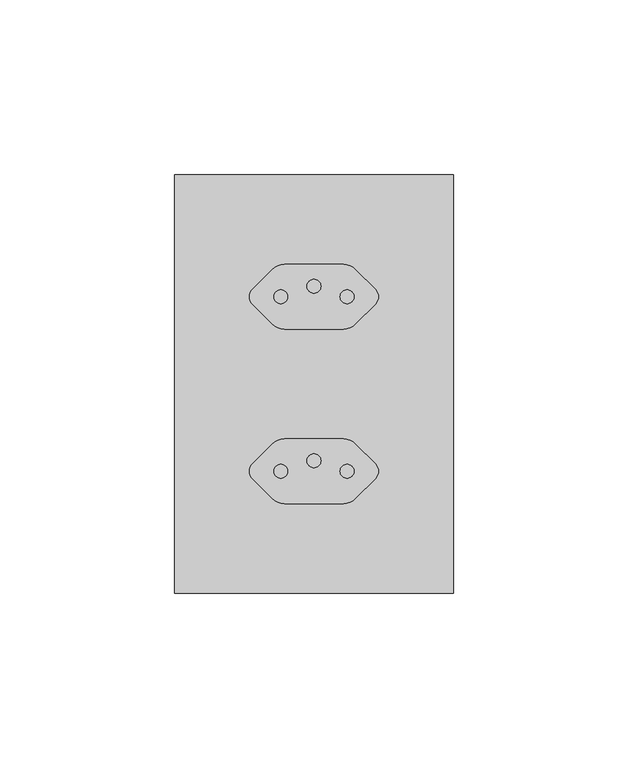
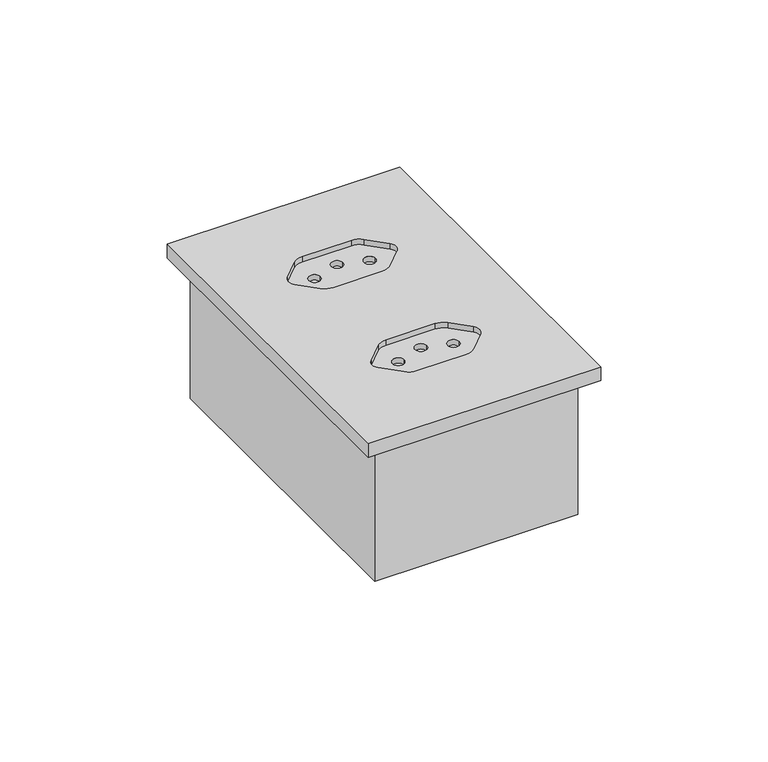
"""IFC4 building model written with IfcOpenShell, lengths in millimetres: proxy geometry, CAIXA VERTICE V7 : Tomada 10A 2s."""

from ifc_helpers import new_model, si_unit, frame, origin, place, context, project, spatial, polyline, circle_curve, faceted_brep, source, transform, mapped, element, save
from ifc_brep_helpers import plane_surface, revolved_surface, advanced_brep


def electrical_fixtures_84a19cd9(model_context):
    return source(origin(), model_context, "Body", "SolidModel", [
        faceted_brep([(33.0, 947.0, -48.0), (33.0, 1053.0, -48.0), (-33.0, 1053.0, -48.0), (-33.0, 947.0, -48.0), (35.0, 1055.0, -50.0), (35.0, 945.0, -50.0), (-35.0, 945.0, -50.0), (-35.0, 1055.0, -50.0), (-35.0, 1055.0, 0.0), (35.0, 1055.0, 0.0), (-35.0, 945.0, 0.0), (35.0, 945.0, 0.0), (33.0, 1053.0, 0.0), (33.0, 947.0, 0.0), (-33.0, 947.0, 0.0), (-33.0, 1053.0, 0.0)], [[[0, 1, 2, 3]], [[4, 5, 6, 7]], [[4, 7, 8, 9]], [[8, 7, 6, 10]], [[10, 6, 5, 11]], [[11, 5, 4, 9]], [[9, 8, 10, 11], [12, 13, 14, 15]], [[13, 12, 1, 0]], [[14, 13, 0, 3]], [[15, 14, 3, 2]], [[12, 15, 2, 1]]]),
        advanced_brep(
        [(40.0, 1060.0, 5.0), (-40.0, 1060.0, 5.0), (-40.0, 940.0, 5.0), (40.0, 940.0, 5.0), (8.4215729, 1015.75, 5.0), (-8.4215729, 1015.75, 5.0), (-11.9571068, 1017.2144661, 5.0), (-17.6213203, 1022.8786797, 5.0), (-17.6213203, 1027.1213203, 5.0), (-11.9571068, 1032.7855339, 5.0), (-8.4215729, 1034.25, 5.0), (8.4215729, 1034.25, 5.0), (11.9571068, 1032.7855339, 5.0), (17.6213203, 1027.1213203, 5.0), (17.6213203, 1022.8786797, 5.0), (11.9571068, 1017.2144661, 5.0), (8.4215729, 965.75, 5.0), (-8.4215729, 965.75, 5.0), (-11.9571068, 967.2144661, 5.0), (-17.6213203, 972.8786797, 5.0), (-17.6213203, 977.1213203, 5.0), (-11.9571068, 982.7855339, 5.0), (-8.4215729, 984.25, 5.0), (8.4215729, 984.25, 5.0), (11.9571068, 982.7855339, 5.0), (17.6213203, 977.1213203, 5.0), (17.6213203, 972.8786797, 5.0), (11.9571068, 967.2144661, 5.0), (-40.0, 1060.0, 0.0), (40.0, 1060.0, 0.0), (40.0, 940.0, 0.0), (-40.0, 940.0, 0.0), (8.4215729, 1015.75, 3.0), (11.9571068, 1017.2144661, 3.0), (17.6213203, 1022.8786797, 3.0), (17.6213203, 1027.1213203, 3.0), (11.9571068, 1032.7855339, 3.0), (8.4215729, 1034.25, 3.0), (-8.4215729, 1034.25, 3.0), (-11.9571068, 1032.7855339, 3.0), (-17.6213203, 1027.1213203, 3.0), (-17.6213203, 1022.8786797, 3.0), (-11.9571068, 1017.2144661, 3.0), (-8.4215729, 1015.75, 3.0), (-7.5, 1025.0, 3.0), (-11.5, 1025.0, 3.0), (11.5, 1025.0, 3.0), (7.5, 1025.0, 3.0), (2.0, 1028.0, 3.0), (-2.0, 1028.0, 3.0), (-11.5, 1025.0, 1.0), (-7.5, 1025.0, 1.0), (7.5, 1025.0, 1.0), (11.5, 1025.0, 1.0), (-2.0, 1028.0, 1.0), (2.0, 1028.0, 1.0), (8.4215729, 965.75, 3.0), (11.9571068, 967.2144661, 3.0), (17.6213203, 972.8786797, 3.0), (17.6213203, 977.1213203, 3.0), (11.9571068, 982.7855339, 3.0), (8.4215729, 984.25, 3.0), (-8.4215729, 984.25, 3.0), (-11.9571068, 982.7855339, 3.0), (-17.6213203, 977.1213203, 3.0), (-17.6213203, 972.8786797, 3.0), (-11.9571068, 967.2144661, 3.0), (-8.4215729, 965.75, 3.0), (-7.5, 975.0, 3.0), (-11.5, 975.0, 3.0), (11.5, 975.0, 3.0), (7.5, 975.0, 3.0), (2.0, 978.0, 3.0), (-2.0, 978.0, 3.0), (-11.5, 975.0, 1.0), (-7.5, 975.0, 1.0), (7.5, 975.0, 1.0), (11.5, 975.0, 1.0), (-2.0, 978.0, 1.0), (2.0, 978.0, 1.0)],
        [
            (0, 1),
            (1, 2),
            (2, 3),
            (3, 0),
            (4, 5),
            (5, 6, circle_curve(frame((-8.4215729, 1020.75, 5.0), z_axis=(0.0, 0.0, -1.0), x_axis=(-1.0, 0.0, 0.0)), 5.0)),
            (6, 7),
            (7, 8, circle_curve(frame((-15.5, 1025.0, 5.0), z_axis=(0.0, 0.0, -1.0), x_axis=(-1.0, 0.0, 0.0)), 3.0)),
            (8, 9),
            (9, 10, circle_curve(frame((-8.4215729, 1029.25, 5.0), z_axis=(0.0, 0.0, -1.0), x_axis=(-1.0, 0.0, 0.0)), 5.0)),
            (10, 11),
            (11, 12, circle_curve(frame((8.4215729, 1029.25, 5.0), z_axis=(0.0, 0.0, -1.0), x_axis=(-1.0, 0.0, 0.0)), 5.0)),
            (12, 13),
            (13, 14, circle_curve(frame((15.5, 1025.0, 5.0), z_axis=(0.0, 0.0, -1.0), x_axis=(-1.0, 0.0, 0.0)), 3.0)),
            (14, 15),
            (15, 4, circle_curve(frame((8.4215729, 1020.75, 5.0), z_axis=(0.0, 0.0, -1.0), x_axis=(-1.0, 0.0, 0.0)), 5.0)),
            (16, 17),
            (17, 18, circle_curve(frame((-8.4215729, 970.75, 5.0), z_axis=(0.0, 0.0, -1.0), x_axis=(-1.0, 0.0, 0.0)), 5.0)),
            (18, 19),
            (19, 20, circle_curve(frame((-15.5, 975.0, 5.0), z_axis=(0.0, 0.0, -1.0), x_axis=(-1.0, 0.0, 0.0)), 3.0)),
            (20, 21),
            (21, 22, circle_curve(frame((-8.4215729, 979.25, 5.0), z_axis=(0.0, 0.0, -1.0), x_axis=(-1.0, 0.0, 0.0)), 5.0)),
            (22, 23),
            (23, 24, circle_curve(frame((8.4215729, 979.25, 5.0), z_axis=(0.0, 0.0, -1.0), x_axis=(-1.0, 0.0, 0.0)), 5.0)),
            (24, 25),
            (25, 26, circle_curve(frame((15.5, 975.0, 5.0), z_axis=(0.0, 0.0, -1.0), x_axis=(-1.0, 0.0, 0.0)), 3.0)),
            (26, 27),
            (27, 16, circle_curve(frame((8.4215729, 970.75, 5.0), z_axis=(0.0, 0.0, -1.0), x_axis=(-1.0, 0.0, 0.0)), 5.0)),
            (28, 29),
            (29, 30),
            (30, 31),
            (31, 28),
            (0, 29),
            (28, 1),
            (31, 2),
            (30, 3),
            (32, 33, circle_curve(frame((8.4215729, 1020.75, 3.0), z_axis=(0.0, 0.0, 1.0), x_axis=(-1.0, 0.0, 0.0)), 5.0)),
            (33, 34),
            (34, 35, circle_curve(frame((15.5, 1025.0, 3.0), z_axis=(0.0, 0.0, 1.0), x_axis=(-1.0, 0.0, 0.0)), 3.0)),
            (35, 36),
            (36, 37, circle_curve(frame((8.4215729, 1029.25, 3.0), z_axis=(0.0, 0.0, 1.0), x_axis=(-1.0, 0.0, 0.0)), 5.0)),
            (37, 38),
            (38, 39, circle_curve(frame((-8.4215729, 1029.25, 3.0), z_axis=(0.0, 0.0, 1.0), x_axis=(-1.0, 0.0, 0.0)), 5.0)),
            (39, 40),
            (40, 41, circle_curve(frame((-15.5, 1025.0, 3.0), z_axis=(0.0, 0.0, 1.0), x_axis=(-1.0, 0.0, 0.0)), 3.0)),
            (41, 42),
            (42, 43, circle_curve(frame((-8.4215729, 1020.75, 3.0), z_axis=(0.0, 0.0, 1.0), x_axis=(-1.0, 0.0, 0.0)), 5.0)),
            (43, 32),
            (44, 45, circle_curve(frame((-9.5, 1025.0, 3.0), z_axis=(0.0, 0.0, -1.0), x_axis=(1.0, 2.301812013077709e-12, 0.0)), 2.0)),
            (45, 44, circle_curve(frame((-9.5, 1025.0, 3.0), z_axis=(0.0, 0.0, -1.0), x_axis=(1.0, 2.301812013077709e-12, 0.0)), 2.0)),
            (46, 47, circle_curve(frame((9.5, 1025.0, 3.0), z_axis=(0.0, 0.0, -1.0), x_axis=(1.0, 2.301812013077709e-12, 0.0)), 2.0)),
            (47, 46, circle_curve(frame((9.5, 1025.0, 3.0), z_axis=(0.0, 0.0, -1.0), x_axis=(1.0, 2.301812013077709e-12, 0.0)), 2.0)),
            (48, 49, circle_curve(frame((0.0, 1028.0, 3.0), z_axis=(0.0, 0.0, -1.0), x_axis=(1.0, 2.301812013077709e-12, 0.0)), 2.0)),
            (49, 48, circle_curve(frame((0.0, 1028.0, 3.0), z_axis=(0.0, 0.0, -1.0), x_axis=(1.0, 2.301812013077709e-12, 0.0)), 2.0)),
            (43, 5),
            (4, 32),
            (42, 6),
            (41, 7),
            (40, 8),
            (39, 9),
            (38, 10),
            (37, 11),
            (36, 12),
            (35, 13),
            (34, 14),
            (33, 15),
            (50, 51, circle_curve(frame((-9.5, 1025.0, 1.0), z_axis=(0.0, 0.0, 1.0), x_axis=(1.0, 2.301812013077709e-12, 0.0)), 2.0)),
            (51, 50, circle_curve(frame((-9.5, 1025.0, 1.0), z_axis=(0.0, 0.0, 1.0), x_axis=(1.0, 2.301812013077709e-12, 0.0)), 2.0)),
            (52, 53, circle_curve(frame((9.5, 1025.0, 1.0), z_axis=(0.0, 0.0, 1.0), x_axis=(1.0, 2.301812013077709e-12, 0.0)), 2.0)),
            (53, 52, circle_curve(frame((9.5, 1025.0, 1.0), z_axis=(0.0, 0.0, 1.0), x_axis=(1.0, 2.301812013077709e-12, 0.0)), 2.0)),
            (54, 55, circle_curve(frame((0.0, 1028.0, 1.0), z_axis=(0.0, 0.0, 1.0), x_axis=(1.0, 2.301812013077709e-12, 0.0)), 2.0)),
            (55, 54, circle_curve(frame((0.0, 1028.0, 1.0), z_axis=(0.0, 0.0, 1.0), x_axis=(1.0, 2.301812013077709e-12, 0.0)), 2.0)),
            (44, 51),
            (50, 45),
            (46, 53),
            (52, 47),
            (48, 55),
            (54, 49),
            (56, 57, circle_curve(frame((8.4215729, 970.75, 3.0), z_axis=(0.0, 0.0, 1.0), x_axis=(-1.0, 0.0, 0.0)), 5.0)),
            (57, 58),
            (58, 59, circle_curve(frame((15.5, 975.0, 3.0), z_axis=(0.0, 0.0, 1.0), x_axis=(-1.0, 0.0, 0.0)), 3.0)),
            (59, 60),
            (60, 61, circle_curve(frame((8.4215729, 979.25, 3.0), z_axis=(0.0, 0.0, 1.0), x_axis=(-1.0, 0.0, 0.0)), 5.0)),
            (61, 62),
            (62, 63, circle_curve(frame((-8.4215729, 979.25, 3.0), z_axis=(0.0, 0.0, 1.0), x_axis=(-1.0, 0.0, 0.0)), 5.0)),
            (63, 64),
            (64, 65, circle_curve(frame((-15.5, 975.0, 3.0), z_axis=(0.0, 0.0, 1.0), x_axis=(-1.0, 0.0, 0.0)), 3.0)),
            (65, 66),
            (66, 67, circle_curve(frame((-8.4215729, 970.75, 3.0), z_axis=(0.0, 0.0, 1.0), x_axis=(-1.0, 0.0, 0.0)), 5.0)),
            (67, 56),
            (68, 69, circle_curve(frame((-9.5, 975.0, 3.0), z_axis=(0.0, 0.0, -1.0), x_axis=(1.0, 2.301812013077709e-12, 0.0)), 2.0)),
            (69, 68, circle_curve(frame((-9.5, 975.0, 3.0), z_axis=(0.0, 0.0, -1.0), x_axis=(1.0, 2.301812013077709e-12, 0.0)), 2.0)),
            (70, 71, circle_curve(frame((9.5, 975.0, 3.0), z_axis=(0.0, 0.0, -1.0), x_axis=(1.0, 2.301812013077709e-12, 0.0)), 2.0)),
            (71, 70, circle_curve(frame((9.5, 975.0, 3.0), z_axis=(0.0, 0.0, -1.0), x_axis=(1.0, 2.301812013077709e-12, 0.0)), 2.0)),
            (72, 73, circle_curve(frame((0.0, 978.0, 3.0), z_axis=(0.0, 0.0, -1.0), x_axis=(1.0, 2.301812013077709e-12, 0.0)), 2.0)),
            (73, 72, circle_curve(frame((0.0, 978.0, 3.0), z_axis=(0.0, 0.0, -1.0), x_axis=(1.0, 2.301812013077709e-12, 0.0)), 2.0)),
            (67, 17),
            (16, 56),
            (66, 18),
            (65, 19),
            (64, 20),
            (63, 21),
            (62, 22),
            (61, 23),
            (60, 24),
            (59, 25),
            (58, 26),
            (57, 27),
            (74, 75, circle_curve(frame((-9.5, 975.0, 1.0), z_axis=(0.0, 0.0, 1.0), x_axis=(1.0, 2.301812013077709e-12, 0.0)), 2.0)),
            (75, 74, circle_curve(frame((-9.5, 975.0, 1.0), z_axis=(0.0, 0.0, 1.0), x_axis=(1.0, 2.301812013077709e-12, 0.0)), 2.0)),
            (76, 77, circle_curve(frame((9.5, 975.0, 1.0), z_axis=(0.0, 0.0, 1.0), x_axis=(1.0, 2.301812013077709e-12, 0.0)), 2.0)),
            (77, 76, circle_curve(frame((9.5, 975.0, 1.0), z_axis=(0.0, 0.0, 1.0), x_axis=(1.0, 2.301812013077709e-12, 0.0)), 2.0)),
            (78, 79, circle_curve(frame((0.0, 978.0, 1.0), z_axis=(0.0, 0.0, 1.0), x_axis=(1.0, 2.301812013077709e-12, 0.0)), 2.0)),
            (79, 78, circle_curve(frame((0.0, 978.0, 1.0), z_axis=(0.0, 0.0, 1.0), x_axis=(1.0, 2.301812013077709e-12, 0.0)), 2.0)),
            (68, 75),
            (74, 69),
            (70, 77),
            (76, 71),
            (72, 79),
            (78, 73),
        ],
        [
            plane_surface(frame((-60.0, 1060.0, 5.0), z_axis=(0.0, 0.0, 1.0), x_axis=(-1.0, 0.0, 0.0))),
            plane_surface(frame((-60.0, 1060.0, 0.0), z_axis=(0.0, 0.0, -1.0), x_axis=(1.0, 0.0, 0.0))),
            plane_surface(frame((40.0, 1060.0, 5.0), z_axis=(0.0, 1.0, 0.0), x_axis=(0.0, 0.0, -1.0))),
            plane_surface(frame((-40.0, 1060.0, 5.0), z_axis=(-1.0, 0.0, 0.0), x_axis=(0.0, 0.0, -1.0))),
            plane_surface(frame((-40.0, 940.0, 5.0), z_axis=(0.0, -1.0, 0.0), x_axis=(0.0, 0.0, -1.0))),
            plane_surface(frame((40.0, 940.0, 5.0), z_axis=(1.0, 0.0, 0.0), x_axis=(0.0, 0.0, -1.0))),
            plane_surface(frame((3.4215729, 1020.75, 3.0), z_axis=(0.0, 0.0, 1.0), x_axis=(0.0, 1.0, 0.0))),
            plane_surface(frame((-8.4215729, 1015.75, 5.0), z_axis=(0.0, 1.0, 0.0), x_axis=(0.0, 0.0, -1.0))),
            revolved_surface(polyline([(-13.4215729, 1020.75, 5.0), (-13.4215729, 1020.75, 3.0)]), (-8.4215729, 1020.75, 3.0), (0.0, 0.0, 1.0)),
            plane_surface(frame((-17.6213203, 1022.8786797, 5.0), z_axis=(0.7071067811865045, 0.7071067811865905, 0.0), x_axis=(0.0, 0.0, -1.0))),
            revolved_surface(polyline([(-18.5, 1025.0, 5.0), (-18.5, 1025.0, 3.0)]), (-15.5, 1025.0, 3.0), (0.0, 0.0, 1.0)),
            plane_surface(frame((-11.9571068, 1032.7855339, 5.0), z_axis=(0.7071067811865515, -0.7071067811865437, 0.0), x_axis=(0.0, 0.0, -1.0))),
            revolved_surface(polyline([(-13.4215729, 1029.25, 5.0), (-13.4215729, 1029.25, 3.0)]), (-8.4215729, 1029.25, 3.0), (0.0, 0.0, 1.0)),
            plane_surface(frame((8.4215729, 1034.25, 5.0), z_axis=(0.0, -1.0, 0.0), x_axis=(0.0, 0.0, -1.0))),
            revolved_surface(polyline([(3.4215728999999993, 1029.25, 5.0), (3.4215728999999993, 1029.25, 3.0)]), (8.4215729, 1029.25, 3.0), (0.0, 0.0, 1.0)),
            plane_surface(frame((17.6213203, 1027.1213203, 5.0), z_axis=(-0.7071067811865307, -0.7071067811865643, 0.0), x_axis=(0.0, 0.0, -1.0))),
            revolved_surface(polyline([(12.5, 1025.0, 5.0), (12.5, 1025.0, 3.0)]), (15.5, 1025.0, 3.0), (0.0, 0.0, 1.0)),
            plane_surface(frame((11.9571068, 1017.2144661, 5.0), z_axis=(-0.7071067811865893, 0.7071067811865058, 0.0), x_axis=(0.0, 0.0, -1.0))),
            revolved_surface(polyline([(3.4215728999999993, 1020.75, 5.0), (3.4215728999999993, 1020.75, 3.0)]), (8.4215729, 1020.75, 3.0), (0.0, 0.0, 1.0)),
            plane_surface(frame((-7.5, 1025.0, 1.0), z_axis=(0.0, 0.0, 1.0), x_axis=(2.301812013077709e-12, -1.0, 0.0))),
            revolved_surface(polyline([(-7.5, 1025.0000000000045, 3.0), (-7.5, 1025.0000000000045, 1.0)]), (-9.5, 1025.0, 1.0), (0.0, 0.0, 1.0)),
            revolved_surface(polyline([(11.5, 1025.0000000000045, 3.0), (11.5, 1025.0000000000045, 1.0)]), (9.5, 1025.0, 5.0), (0.0, 0.0, 1.0)),
            revolved_surface(polyline([(2.0, 1028.0000000000045, 3.0), (2.0, 1028.0000000000045, 1.0)]), (0.0, 1028.0, 5.0), (0.0, 0.0, 1.0)),
            plane_surface(frame((3.4215729, 970.75, 3.0), z_axis=(0.0, 0.0, 1.0), x_axis=(0.0, 1.0, 0.0))),
            plane_surface(frame((-8.4215729, 965.75, 5.0), z_axis=(0.0, 1.0, 0.0), x_axis=(0.0, 0.0, -1.0))),
            revolved_surface(polyline([(-13.4215729, 970.75, 5.0), (-13.4215729, 970.75, 3.0)]), (-8.4215729, 970.75, 3.0), (0.0, 0.0, 1.0)),
            plane_surface(frame((-17.6213203, 972.8786797, 5.0), z_axis=(0.7071067811865045, 0.7071067811865905, 0.0), x_axis=(0.0, 0.0, -1.0))),
            revolved_surface(polyline([(-18.5, 975.0, 5.0), (-18.5, 975.0, 3.0)]), (-15.5, 975.0, 3.0), (0.0, 0.0, 1.0)),
            plane_surface(frame((-11.9571068, 982.7855339, 5.0), z_axis=(0.7071067811865515, -0.7071067811865437, 0.0), x_axis=(0.0, 0.0, -1.0))),
            revolved_surface(polyline([(-13.4215729, 979.25, 5.0), (-13.4215729, 979.25, 3.0)]), (-8.4215729, 979.25, 3.0), (0.0, 0.0, 1.0)),
            plane_surface(frame((8.4215729, 984.25, 5.0), z_axis=(0.0, -1.0, 0.0), x_axis=(0.0, 0.0, -1.0))),
            revolved_surface(polyline([(3.4215728999999993, 979.25, 5.0), (3.4215728999999993, 979.25, 3.0)]), (8.4215729, 979.25, 3.0), (0.0, 0.0, 1.0)),
            plane_surface(frame((17.6213203, 977.1213203, 5.0), z_axis=(-0.7071067811865307, -0.7071067811865643, 0.0), x_axis=(0.0, 0.0, -1.0))),
            revolved_surface(polyline([(12.5, 975.0, 5.0), (12.5, 975.0, 3.0)]), (15.5, 975.0, 3.0), (0.0, 0.0, 1.0)),
            plane_surface(frame((11.9571068, 967.2144661, 5.0), z_axis=(-0.7071067811865893, 0.7071067811865058, 0.0), x_axis=(0.0, 0.0, -1.0))),
            revolved_surface(polyline([(3.4215728999999993, 970.75, 5.0), (3.4215728999999993, 970.75, 3.0)]), (8.4215729, 970.75, 3.0), (0.0, 0.0, 1.0)),
            plane_surface(frame((-7.5, 975.0, 1.0), z_axis=(0.0, 0.0, 1.0), x_axis=(2.301812013077709e-12, -1.0, 0.0))),
            revolved_surface(polyline([(-7.5, 975.0000000000045, 3.0), (-7.5, 975.0000000000045, 1.0)]), (-9.5, 975.0, 1.0), (0.0, 0.0, 1.0)),
            revolved_surface(polyline([(11.5, 975.0000000000045, 3.0), (11.5, 975.0000000000045, 1.0)]), (9.5, 975.0, 5.0), (0.0, 0.0, 1.0)),
            revolved_surface(polyline([(2.0, 978.0000000000045, 3.0), (2.0, 978.0000000000045, 1.0)]), (0.0, 978.0, 5.0), (0.0, 0.0, 1.0)),
        ],
        [
            (0, [[1, 2, 3, 4], [5, 6, 7, 8, 9, 10, 11, 12, 13, 14, 15, 16], [17, 18, 19, 20, 21, 22, 23, 24, 25, 26, 27, 28]]),
            (1, [[29, 30, 31, 32]]),
            (2, [[-1, 33, -29, 34]]),
            (3, [[-2, -34, -32, 35]]),
            (4, [[-3, -35, -31, 36]]),
            (5, [[-4, -36, -30, -33]]),
            (6, [[37, 38, 39, 40, 41, 42, 43, 44, 45, 46, 47, 48], [49, 50], [51, 52], [53, 54]]),
            (7, [[-48, 55, -5, 56]]),
            (8, [[-47, 57, -6, -55]]),
            (9, [[-46, 58, -7, -57]]),
            (10, [[-45, 59, -8, -58]]),
            (11, [[-44, 60, -9, -59]]),
            (12, [[-43, 61, -10, -60]]),
            (13, [[-42, 62, -11, -61]]),
            (14, [[-41, 63, -12, -62]]),
            (15, [[-40, 64, -13, -63]]),
            (16, [[-39, 65, -14, -64]]),
            (17, [[-38, 66, -15, -65]]),
            (18, [[-37, -56, -16, -66]]),
            (19, [[67, 68]]),
            (19, [[69, 70]]),
            (19, [[71, 72]]),
            (20, [[-49, 73, -67, 74]]),
            (20, [[-50, -74, -68, -73]]),
            (21, [[-51, 75, -69, 76]]),
            (21, [[-52, -76, -70, -75]]),
            (22, [[-53, 77, -71, 78]]),
            (22, [[-54, -78, -72, -77]]),
            (23, [[79, 80, 81, 82, 83, 84, 85, 86, 87, 88, 89, 90], [91, 92], [93, 94], [95, 96]]),
            (24, [[-90, 97, -17, 98]]),
            (25, [[-89, 99, -18, -97]]),
            (26, [[-88, 100, -19, -99]]),
            (27, [[-87, 101, -20, -100]]),
            (28, [[-86, 102, -21, -101]]),
            (29, [[-85, 103, -22, -102]]),
            (30, [[-84, 104, -23, -103]]),
            (31, [[-83, 105, -24, -104]]),
            (32, [[-82, 106, -25, -105]]),
            (33, [[-81, 107, -26, -106]]),
            (34, [[-80, 108, -27, -107]]),
            (35, [[-79, -98, -28, -108]]),
            (36, [[109, 110]]),
            (36, [[111, 112]]),
            (36, [[113, 114]]),
            (37, [[-91, 115, -109, 116]]),
            (37, [[-92, -116, -110, -115]]),
            (38, [[-93, 117, -111, 118]]),
            (38, [[-94, -118, -112, -117]]),
            (39, [[-95, 119, -113, 120]]),
            (39, [[-96, -120, -114, -119]]),
        ],
    ),
    ])


if __name__ == "__main__":
    model = new_model("IFC4")
    model_context = context("Model", 3, world=origin())
    ifc_project = project(units=[si_unit("LENGTHUNIT", "METRE", prefix="MILLI")], contexts=[model_context])
    site = spatial("IfcSite", under=ifc_project)
    building = spatial("IfcBuilding", under=site)
    placement = place(None, origin())
    electrical_fixtures_shape = electrical_fixtures_84a19cd9(model_context)
    element("IfcBuildingElementProxy", 1, Name="CAIXA VERTICE V7 : Tomada 10A 2s", ObjectType="CAIXA VERTICE V7 : Tomada 10A 2s", at=placement, inside=building, context=model_context, shape_type="MappedRepresentation", body=[
        mapped(electrical_fixtures_shape, transform((0.0, 0.0, 0.0), x_axis=(1.0, 0.0, 0.0), y_axis=(0.0, 1.0, 0.0), z_axis=(0.0, 0.0, 1.0))),
    ])
    save(model, "model.ifc")

# Revit data of these elements
# Type "CAIXA VERTICE V7 : Tomada 10A 2s"
#   URL = "www.facebook.com/verticetreinamentos"
#   SEÇÃO [instance default] = ""
#   Rotação [instance default] = 0.00°
#   LARGURA DA TAMPA = 0.08 m
#   BORDA = 0.01 m
#   ALTURA DE INSTALAÇÃO [instance default] = 1.10 m
#   Distância Anotação [instance default] = 0.0015 m
#   ALTURA DA TAMPA = 0.12 m
#   Vertical [instance default] = yes
#   VER SEÇÃO [instance default] = no
#   SHADE ESQ [instance default] = no
#   SHADE DIR [instance default] = yes
#   HORIZONTAL [instance default] = no
#   ANDAR COM A LEGENDA [instance default] = 0
#   Material Tampa [instance default] = Plástico, branco opaco
#   Caixa = element 1798515
#   Anotação = element 1798529
#   Default Elevation = 0
# Element 1 (IfcBuildingElementProxy, "CAIXA VERTICE V7 : Tomada 10A 2s")
#   ALTURA DE INSTALAÇÃO = 1.00 m
#   Materials on its faces: "Plástico, branco opaco"
# Materials
#   "Plástico, branco opaco": class "Plástico", colour RGB 120 120 120, transparency 0, Description = "Plastic, generic, opaque white", Cost = 0
